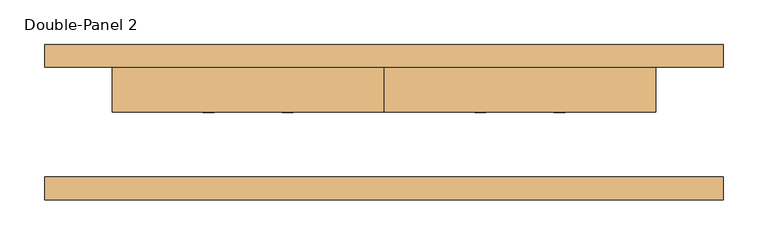
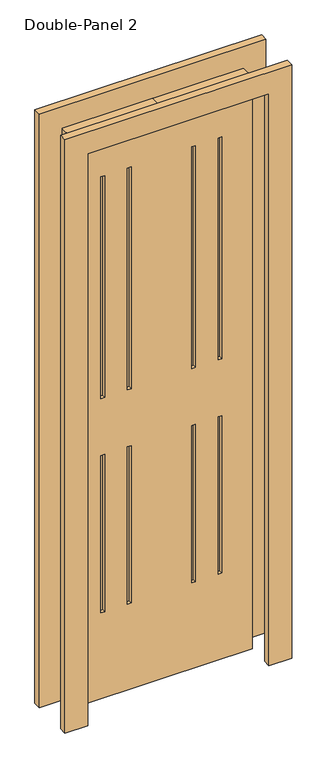
"""IFC4 building model written with IfcOpenShell, lengths in millimetres: door geometry, Double-Panel 2."""

from ifc_helpers import new_model, si_unit, frame, origin, place, context, project, spatial, polyline, outline, extrude, source, transform, mapped, element, save


def double_panel_2_437d2bf6(model_context):
    return source(origin(), model_context, "Body", "SweptSolid", [
        extrude(outline(polyline([(2108.2, -381.0), (0.0, -381.0), (0.0, -304.8), (2032.0, -304.8), (2032.0, 304.8), (0.0, 304.8), (0.0, 381.0), (2108.2, 381.0), (2108.2, -381.0)])), frame((0.0, 61.9125, 0.0), z_axis=(0.0, 1.0, 0.0), x_axis=(0.0, 0.0, 1.0)), (0.0, 0.0, 1.0), 25.4),
        extrude(outline(polyline([(190.5, 49.2125), (203.2, 49.2125), (203.2, 23.8125), (190.5, 23.8125), (190.5, 49.2125)])), frame((0.0, 0.0, 1066.8), z_axis=(0.0, 0.0, 1.0), x_axis=(1.0, 0.0, 0.0)), (0.0, 0.0, 1.0), 787.4),
        extrude(outline(polyline([(101.6, 49.2125), (114.3, 49.2125), (114.3, 23.8125), (101.6, 23.8125), (101.6, 49.2125)])), frame((0.0, 0.0, 1066.8), z_axis=(0.0, 0.0, 1.0), x_axis=(1.0, 0.0, 0.0)), (0.0, 0.0, 1.0), 787.4),
        extrude(outline(polyline([(190.5, 49.2125), (203.2, 49.2125), (203.2, 23.8125), (190.5, 23.8125), (190.5, 49.2125)])), frame((0.0, 0.0, 304.8), z_axis=(0.0, 0.0, 1.0), x_axis=(1.0, 0.0, 0.0)), (0.0, 0.0, 1.0), 558.8),
        extrude(outline(polyline([(101.6, 49.2125), (114.3, 49.2125), (114.3, 23.8125), (101.6, 23.8125), (101.6, 49.2125)])), frame((0.0, 0.0, 304.8), z_axis=(0.0, 0.0, 1.0), x_axis=(1.0, 0.0, 0.0)), (0.0, 0.0, 1.0), 558.8),
        extrude(outline(polyline([(-114.3, 49.2125), (-101.6, 49.2125), (-101.6, 23.8125), (-114.3, 23.8125), (-114.3, 49.2125)])), frame((0.0, 0.0, 1066.8), z_axis=(0.0, 0.0, 1.0), x_axis=(1.0, 0.0, 0.0)), (0.0, 0.0, 1.0), 787.4),
        extrude(outline(polyline([(-203.2, 49.2125), (-190.5, 49.2125), (-190.5, 23.8125), (-203.2, 23.8125), (-203.2, 49.2125)])), frame((0.0, 0.0, 1066.8), z_axis=(0.0, 0.0, 1.0), x_axis=(1.0, 0.0, 0.0)), (0.0, 0.0, 1.0), 787.4),
        extrude(outline(polyline([(-114.3, 49.2125), (-101.6, 49.2125), (-101.6, 23.8125), (-114.3, 23.8125), (-114.3, 49.2125)])), frame((0.0, 0.0, 304.8), z_axis=(0.0, 0.0, 1.0), x_axis=(1.0, 0.0, 0.0)), (0.0, 0.0, 1.0), 558.8),
        extrude(outline(polyline([(-203.2, 49.2125), (-190.5, 49.2125), (-190.5, 23.8125), (-203.2, 23.8125), (-203.2, 49.2125)])), frame((0.0, 0.0, 304.8), z_axis=(0.0, 0.0, 1.0), x_axis=(1.0, 0.0, 0.0)), (0.0, 0.0, 1.0), 558.8),
        extrude(outline(polyline([(2032.0, 0.0), (2032.0, -304.8), (0.0, -304.8), (0.0, 0.0), (0.0, 304.8), (2032.0, 304.8), (2032.0, 0.0)]), holes=[polyline([(1854.2, 190.5), (1854.2, 203.2), (1066.8, 203.2), (1066.8, 190.5), (1854.2, 190.5)]), polyline([(1854.2, 101.6), (1854.2, 114.3), (1066.8, 114.3), (1066.8, 101.6), (1854.2, 101.6)]), polyline([(863.6, 190.5), (863.6, 203.2), (304.8, 203.2), (304.8, 190.5), (863.6, 190.5)]), polyline([(863.6, 101.6), (863.6, 114.3), (304.8, 114.3), (304.8, 101.6), (863.6, 101.6)]), polyline([(1066.8, -114.3), (1854.2, -114.3), (1854.2, -101.6), (1066.8, -101.6), (1066.8, -114.3)]), polyline([(1854.2, -203.2), (1854.2, -190.5), (1066.8, -190.5), (1066.8, -203.2), (1854.2, -203.2)]), polyline([(863.6, -114.3), (863.6, -101.6), (304.8, -101.6), (304.8, -114.3), (863.6, -114.3)]), polyline([(863.6, -203.2), (863.6, -190.5), (304.8, -190.5), (304.8, -203.2), (863.6, -203.2)])]), frame((0.0, 11.1125, 0.0), z_axis=(0.0, 1.0, 0.0), x_axis=(0.0, 0.0, 1.0)), (0.0, 0.0, 1.0), 50.8),
        extrude(outline(polyline([(2032.0, -304.8), (2032.0, 304.8), (0.0, 304.8), (0.0, 381.0), (2108.2, 381.0), (2108.2, -381.0), (0.0, -381.0), (0.0, -304.8), (2032.0, -304.8)])), frame((0.0, -87.3125, 0.0), z_axis=(0.0, 1.0, 0.0), x_axis=(0.0, 0.0, 1.0)), (0.0, 0.0, 1.0), 25.4),
    ])


if __name__ == "__main__":
    model = new_model("IFC4")
    model_context = context("Model", 3, world=origin())
    ifc_project = project(units=[si_unit("LENGTHUNIT", "METRE", prefix="MILLI")], contexts=[model_context])
    site = spatial("IfcSite", under=ifc_project)
    building = spatial("IfcBuilding", under=site)
    placement = place(None, origin())
    double_panel_2_shape = double_panel_2_437d2bf6(model_context)
    element("IfcDoor", 1, ObjectType="Double-Panel 2 : 24\" x 80\"  White", at=placement, inside=building, context=model_context, shape_type="MappedRepresentation", body=[
        mapped(double_panel_2_shape, transform((0.0, 0.0, 0.0), x_axis=(1.0, 0.0, 0.0), y_axis=(0.0, 1.0, 0.0), z_axis=(0.0, 0.0, 1.0))),
    ])
    save(model, "model.ifc")

# Revit data of these elements
# Type "Double-Panel 2 : 24\" x 80\"  White"
#   Type Mark = "79"
#   COBie.Type.CreatedBy = "doug.wood@us.ibm.com"
#   COBie.Type.CreatedOn = "2016-04-14T02:07:24"
#   COBie.Type.Name = "Doors_Double-Panel 2_24\" x 80\"  White_79"
#   COBie.Type.Category = "23-30 10 00 : Doors"
#   COBie.Type.Description = "Double-Panel 2_24\" x 80\"  White"
#   COBie.Type.Manufacturer = ""
#   COBie.Type.ModelNumber = ""
#   Construction Type Id = "MDOOR"
#   Assembly Code = "C1020"
#   Analytic Construction = "Metal"
#   COBie.Type.ReplacementCost = 0
#   Thickness = 0' - 2"
#   Heat Transfer Coefficient (U) = 3.7021 W/(m²·K)
#   Height = 6' - 8"
#   Trim Projection Ext = 0' - 1"
#   Trim Projection Int = 0' - 1"
#   Trim Width = 0' - 3"
#   Width = 2' - 0"
#   COBie.Type = no
#   Door Material = Door - Panel
#   Frame Material = Door - Frame - White
#   Visual Light Transmittance = 0
#   Solar Heat Gain Coefficient = 0
#   Function = (empty or 0)
#   Wall Closure = (empty or 0)
# Element 1 (IfcDoor, "Double-Panel 2 : 24\" x 80\"  White")
#   Materials on its faces: "Door - Panel", "Door - Frame - White"
# Materials
#   "Door - Panel": class "Wood", colour RGB 255 255 255, transparency 0, Cost = 0
#   "Door - Frame - White": class "Miscellaneous", colour RGB 255 255 255, transparency 0, Cost = 0
